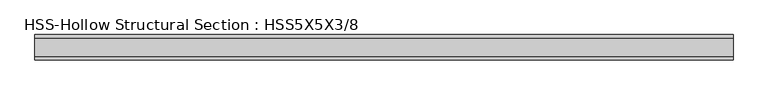
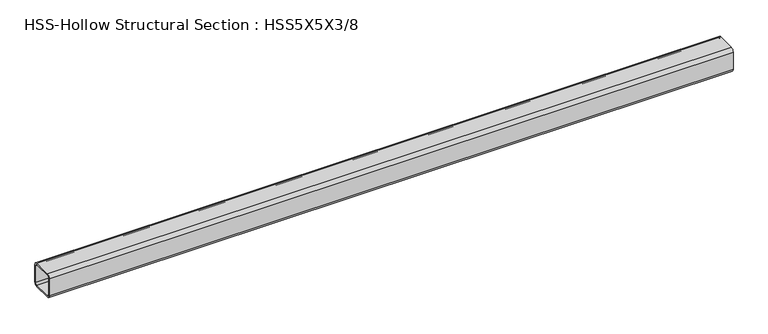
"""IFC4 building model written with IfcOpenShell, lengths in millimetres: member geometry, HSS-Hollow Structural Section : HSS5X5X3/8."""

from ifc_helpers import new_model, si_unit, point, frame, frame_2d, origin, place, context, project, spatial, polyline, circle_curve, trimmed, segment, composite_curve, outline, extrude, source, transform, mapped, element, save


def hss_hollow_structural_section_hss5x5x3_8_885ac686(model_context):
    return source(origin(), model_context, "Body", "SweptSolid", [
        extrude(outline(composite_curve([segment(polyline([(63.5, 45.7708), (63.5, -45.7708)]), True, "CONTINUOUS"), segment(trimmed(circle_curve(frame_2d((45.7708, -45.7708)), 17.7292), [point((63.5, -45.7708))], [point((45.7708, -63.5))], False, "CARTESIAN"), True, "CONTINUOUS"), segment(polyline([(45.7708, -63.5), (-45.7708, -63.5)]), True, "CONTINUOUS"), segment(trimmed(circle_curve(frame_2d((-45.7708, -45.7708)), 17.7292), [point((-45.7708, -63.5))], [point((-63.5, -45.7708))], False, "CARTESIAN"), True, "CONTINUOUS"), segment(polyline([(-63.5, -45.7708), (-63.5, 45.7708)]), True, "CONTINUOUS"), segment(trimmed(circle_curve(frame_2d((-45.7708, 45.7708)), 17.7292), [point((-63.5, 45.7708))], [point((-45.7708, 63.5))], False, "CARTESIAN"), True, "CONTINUOUS"), segment(polyline([(-45.7708, 63.5), (45.7708, 63.5)]), True, "CONTINUOUS"), segment(trimmed(circle_curve(frame_2d((45.7708, 45.7708)), 17.7292), [point((45.7708, 63.5))], [point((63.5, 45.7708))], False, "CARTESIAN"), True, "CONTINUOUS")], self_intersect=False), holes=[composite_curve([segment(trimmed(circle_curve(frame_2d((-45.7708, 45.7708)), 8.8646), [point((-45.7708, 54.6354))], [point((-54.6354, 45.7708))], True, "CARTESIAN"), True, "CONTINUOUS"), segment(polyline([(-54.6354, 45.7708), (-54.6354, -45.7708)]), True, "CONTINUOUS"), segment(trimmed(circle_curve(frame_2d((-45.7708, -45.7708)), 8.8646), [point((-54.6354, -45.7708))], [point((-45.7708, -54.6354))], True, "CARTESIAN"), True, "CONTINUOUS"), segment(polyline([(-45.7708, -54.6354), (45.7708, -54.6354)]), True, "CONTINUOUS"), segment(trimmed(circle_curve(frame_2d((45.7708, -45.7708)), 8.8646), [point((45.7708, -54.6354))], [point((54.6354, -45.7708))], True, "CARTESIAN"), True, "CONTINUOUS"), segment(polyline([(54.6354, -45.7708), (54.6354, 45.7708)]), True, "CONTINUOUS"), segment(trimmed(circle_curve(frame_2d((45.7708, 45.7708)), 8.8646), [point((54.6354, 45.7708))], [point((45.7708, 54.6354))], True, "CARTESIAN"), True, "CONTINUOUS"), segment(polyline([(45.7708, 54.6354), (-45.7708, 54.6354)]), True, "CONTINUOUS")], self_intersect=False)]), frame((-1647.9284414, 0.0, 0.0), z_axis=(1.0, 0.0, 0.0), x_axis=(0.0, 1.0, 0.0)), (0.0, 0.0, 1.0), 3514.3211622),
    ])


if __name__ == "__main__":
    model = new_model("IFC4")
    model_context = context("Model", 3, world=origin())
    ifc_project = project(units=[si_unit("LENGTHUNIT", "METRE", prefix="MILLI")], contexts=[model_context])
    site = spatial("IfcSite", under=ifc_project)
    building = spatial("IfcBuilding", under=site)
    placement = place(None, origin())
    hss_hollow_structural_section_hss5x5x3_8_shape = hss_hollow_structural_section_hss5x5x3_8_885ac686(model_context)
    element("IfcMember", 1, ObjectType="HSS-Hollow Structural Section : HSS5X5X3/8", at=placement, inside=building, context=model_context, shape_type="MappedRepresentation", body=[
        mapped(hss_hollow_structural_section_hss5x5x3_8_shape, transform((0.0, 0.0, 0.0), x_axis=(1.0, 0.0, 0.0), y_axis=(0.0, 1.0, 0.0), z_axis=(0.0, 0.0, 1.0))),
    ])
    save(model, "model.ifc")

# Revit data of these elements
# Type "HSS-Hollow Structural Section : HSS5X5X3/8"
#   Assembly Code = "B10"
#   Shape = "Square"
#   W = 22.3
#   Ht = 0' - 5"
#   Length [instance default] = 5' - 0"
#   b = 0' - 5"
#   kr = 0' - 0.698"
#   t = 0' - 0.349"
#   A = 0.0429167 SF
#   Structural Material [instance default] = Steel ASTM A500, Grade B, Rectangular and Square
# Element 1 (IfcMember, "HSS-Hollow Structural Section : HSS5X5X3/8")
#   Materials on its faces: "Steel ASTM A500, Grade B, Rectangular and Square"
# Materials
#   "Steel ASTM A500, Grade B, Rectangular and Square": class "Metal", colour RGB 199 199 199, transparency 0, Description = "Carbon steel", Cost = 0
